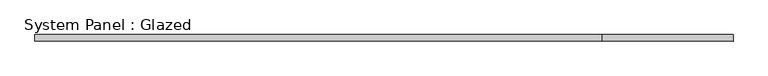
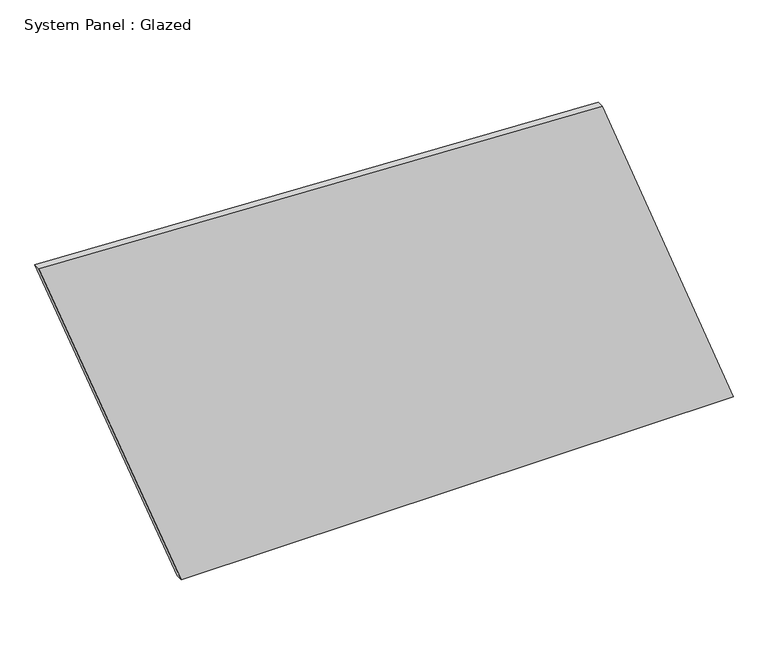
"""IFC4 building model written with IfcOpenShell, lengths in millimetres: plate geometry, System Panel : Glazed."""

from ifc_helpers import new_model, si_unit, frame, origin, place, context, project, spatial, polyline, outline, extrude, source, transform, mapped, element, save


def system_panel_glazed_153f5ef4(model_context):
    return source(origin(), model_context, "Body", "SweptSolid", [
        extrude(outline(polyline([(0.0, -783.8637544), (0.0, 1329.4714835), (1353.0277195, 828.4894888), (1450.3242078, -1329.4714835), (0.0, -783.8637544)])), frame((0.0, -49.5, 0.0), z_axis=(0.0, 1.0, 0.0), x_axis=(0.0, 0.0, 1.0)), (0.0, 0.0, 1.0), 25.0),
    ])


if __name__ == "__main__":
    model = new_model("IFC4")
    model_context = context("Model", 3, world=origin())
    ifc_project = project(units=[si_unit("LENGTHUNIT", "METRE", prefix="MILLI")], contexts=[model_context])
    site = spatial("IfcSite", under=ifc_project)
    building = spatial("IfcBuilding", under=site)
    placement = place(None, origin())
    system_panel_glazed_shape = system_panel_glazed_153f5ef4(model_context)
    element("IfcPlate", 1, ObjectType="System Panel : Glazed", at=placement, inside=building, context=model_context, shape_type="MappedRepresentation", body=[
        mapped(system_panel_glazed_shape, transform((0.0, 0.0, 0.0), x_axis=(1.0, 0.0, 0.0), y_axis=(0.0, 1.0, 0.0), z_axis=(0.0, 0.0, 1.0))),
    ])
    save(model, "model.ifc")

# Revit data of these elements
# Element 1 (IfcPlate, "System Panel : Glazed")
#   Materials on its faces: "Glass, Clear Glazing"
# Materials
#   "Glass, Clear Glazing": class "Glass", colour RGB 247 249 248, transparency 0.85, Description = "Clear glazing", Cost = 0
